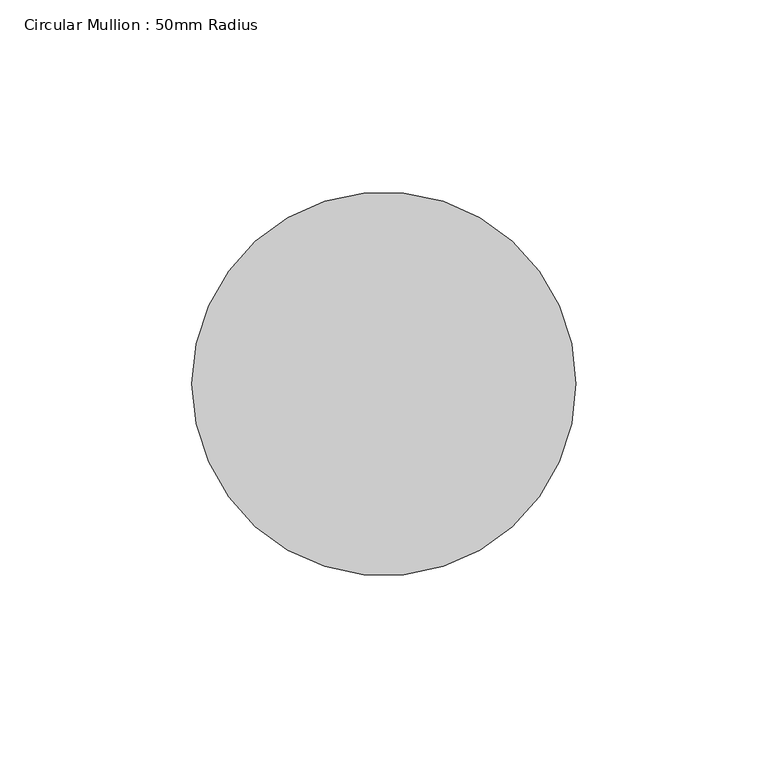
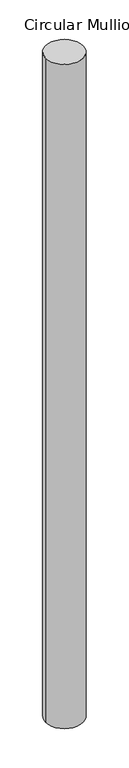
"""IFC4 building model written with IfcOpenShell, lengths in millimetres: member geometry, Circular Mullion : 50mm Radius."""

from ifc_helpers import new_model, si_unit, point, frame, frame_2d, origin, place, context, project, spatial, circle_curve, trimmed, segment, composite_curve, outline, extrude, source, transform, mapped, element, save


def circular_mullion_50mm_radius_bae572da(model_context):
    return source(origin(), model_context, "Body", "SweptSolid", [
        extrude(outline(composite_curve([segment(trimmed(circle_curve(frame_2d((-50.0, 0.0)), 50.0), [point((0.0, 0.0))], [point((-100.0, 0.0))], False, "CARTESIAN"), True, "CONTINUOUS"), segment(trimmed(circle_curve(frame_2d((-50.0, 0.0)), 50.0), [point((-100.0, 0.0))], [point((0.0, 0.0))], False, "CARTESIAN"), True, "CONTINUOUS")], self_intersect=False)), frame((0.0, 0.0, -1866.0435526), z_axis=(0.0, 0.0, 1.0), x_axis=(1.0, 0.0, 0.0)), (0.0, 0.0, 1.0), 1866.0435526),
    ])


if __name__ == "__main__":
    model = new_model("IFC4")
    model_context = context("Model", 3, world=origin())
    ifc_project = project(units=[si_unit("LENGTHUNIT", "METRE", prefix="MILLI")], contexts=[model_context])
    site = spatial("IfcSite", under=ifc_project)
    building = spatial("IfcBuilding", under=site)
    placement = place(None, origin())
    circular_mullion_50mm_radius_shape = circular_mullion_50mm_radius_bae572da(model_context)
    element("IfcMember", 1, ObjectType="Circular Mullion : 50mm Radius", at=placement, inside=building, context=model_context, shape_type="MappedRepresentation", body=[
        mapped(circular_mullion_50mm_radius_shape, transform((0.0, 0.0, 0.0), x_axis=(1.0, 0.0, 0.0), y_axis=(0.0, 1.0, 0.0), z_axis=(0.0, 0.0, 1.0))),
    ])
    save(model, "model.ifc")

# Revit data of these elements
# Type "Circular Mullion : 50mm Radius"
#   built-in parameter 1007350 = 0.164042 (stored number, unit not read)
# Element 1 (IfcMember, "Circular Mullion : 50mm Radius")
#   Materials on its faces: "Aluminium"
# Materials
#   "Aluminium": class "Metal", colour RGB 247 247 247, transparency 0, Description = "Aluminium 6061", Cost = 0
